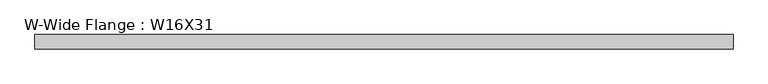
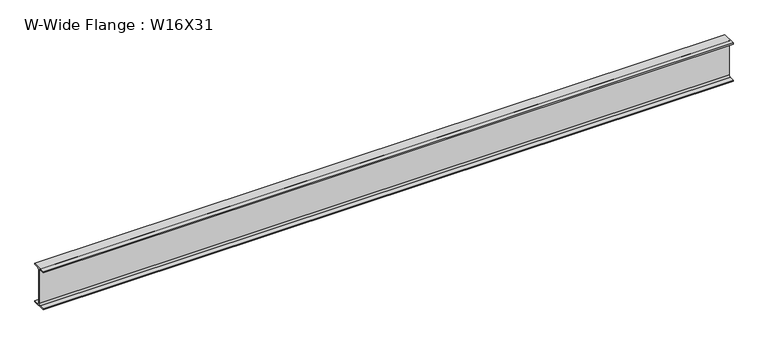
"""IFC4 building model written with IfcOpenShell, lengths in millimetres: beam geometry, W-Wide Flange : W16X31."""

from ifc_helpers import new_model, si_unit, point, frame, frame_2d, origin, place, context, project, spatial, polyline, circle_curve, trimmed, segment, composite_curve, outline, extrude, source, transform, mapped, element, save


def w_wide_flange_w16x31_e9b65252(model_context):
    return source(origin(), model_context, "Body", "SweptSolid", [
        extrude(outline(composite_curve([segment(polyline([(70.231, -190.754), (70.231, -201.93), (-70.231, -201.93), (-70.231, -190.754), (-20.8915, -190.754)]), True, "CONTINUOUS"), segment(trimmed(circle_curve(frame_2d((-20.8915, -173.355)), 17.399), [point((-20.8915, -190.754))], [point((-3.4925, -173.355))], True, "CARTESIAN"), True, "CONTINUOUS"), segment(polyline([(-3.4925, -173.355), (-3.4925, 173.355)]), True, "CONTINUOUS"), segment(trimmed(circle_curve(frame_2d((-20.8915, 173.355)), 17.399), [point((-3.4925, 173.355))], [point((-20.8915, 190.754))], True, "CARTESIAN"), True, "CONTINUOUS"), segment(polyline([(-20.8915, 190.754), (-70.231, 190.754), (-70.231, 201.93), (70.231, 201.93), (70.231, 190.754), (20.8915, 190.754)]), True, "CONTINUOUS"), segment(trimmed(circle_curve(frame_2d((20.8915, 173.355)), 17.399), [point((20.8915, 190.754))], [point((3.4925, 173.355))], True, "CARTESIAN"), True, "CONTINUOUS"), segment(polyline([(3.4925, 173.355), (3.4925, -173.355)]), True, "CONTINUOUS"), segment(trimmed(circle_curve(frame_2d((20.8915, -173.355)), 17.399), [point((3.4925, -173.355))], [point((20.8915, -190.754))], True, "CARTESIAN"), True, "CONTINUOUS"), segment(polyline([(20.8915, -190.754), (70.231, -190.754)]), True, "CONTINUOUS")], self_intersect=False)), frame((-3424.2379887, 0.0, 0.0), z_axis=(1.0, 0.0, 0.0), x_axis=(0.0, 1.0, 0.0)), (0.0, 0.0, 1.0), 6879.267499),
    ])


if __name__ == "__main__":
    model = new_model("IFC4")
    model_context = context("Model", 3, world=origin())
    ifc_project = project(units=[si_unit("LENGTHUNIT", "METRE", prefix="MILLI")], contexts=[model_context])
    site = spatial("IfcSite", under=ifc_project)
    building = spatial("IfcBuilding", under=site)
    placement = place(None, origin())
    w_wide_flange_w16x31_shape = w_wide_flange_w16x31_e9b65252(model_context)
    element("IfcBeam", 1, ObjectType="W-Wide Flange : W16X31", at=placement, inside=building, context=model_context, shape_type="MappedRepresentation", body=[
        mapped(w_wide_flange_w16x31_shape, transform((0.0, 0.0, 0.0), x_axis=(1.0, 0.0, 0.0), y_axis=(0.0, 1.0, 0.0), z_axis=(0.0, 0.0, 1.0))),
    ])
    save(model, "model.ifc")

# Revit data of these elements
# Type "W-Wide Flange : W16X31"
#   Assembly Code = "B10"
#   W = 31
#   Start Extension Calculation [instance default] = 10' - 0"
#   Start Extension [instance default] = -0' - 0 1/2"
#   End Extension Calculation [instance default] = 10' - 0"
#   End Extension [instance default] = -0' - 0 1/2"
#   Length [instance default] = 5' - 0"
#   bf = 0' - 5.53"
#   d = 1' - 3.9"
#   k = 0' - 1 1/8"
#   k2 = 0' - 0.685"
#   tf = 0' - 0.44"
#   tw = 0' - 0.275"
#   A = 0.0634028 SF
#   Beam Material [instance default] = Metal - Steel - ASTM A992
# Element 1 (IfcBeam, "W-Wide Flange : W16X31")
#   Materials on its faces: "Metal - Steel - ASTM A992"
# Materials
#   "Metal - Steel - ASTM A992": class "Metal", colour RGB 128 0 0, transparency 0
